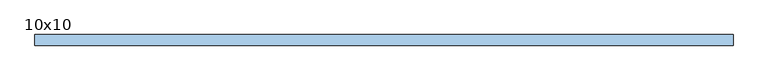
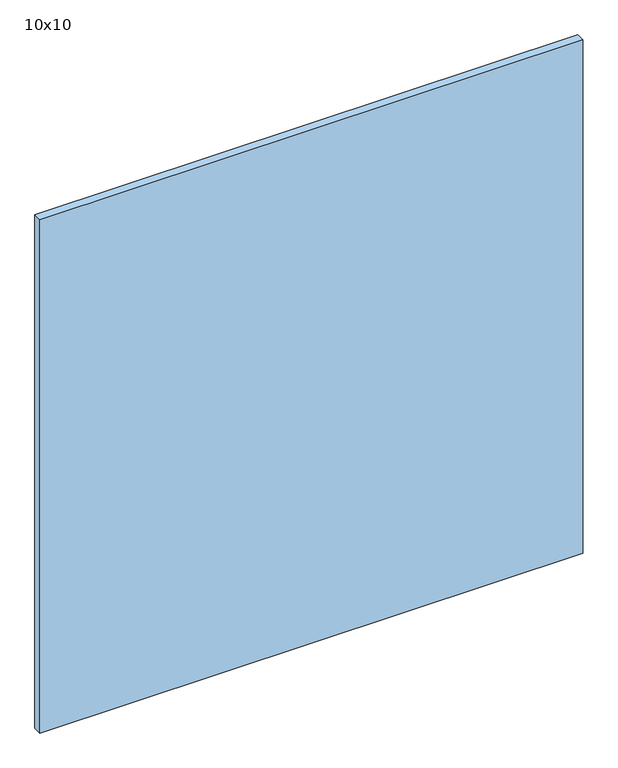
"""IFC4 building model written with IfcOpenShell, lengths in millimetres: window geometry, Window_skiss : 10x10."""

from ifc_helpers import new_model, si_unit, frame, origin, place, context, project, spatial, polyline, outline, extrude, source, transform, mapped, element, save


def window_10x10_03730955(model_context):
    return source(origin(), model_context, "Body", "SweptSolid", [
        extrude(outline(polyline([(575.0, 2.0), (-435.0, 2.0), (-435.0, 18.0), (575.0, 18.0), (575.0, 2.0)])), frame((0.0, 0.0, 800.0), z_axis=(0.0, 0.0, 1.0), x_axis=(1.0, 0.0, 0.0)), (0.0, 0.0, 1.0), 1010.0),
    ])


if __name__ == "__main__":
    model = new_model("IFC4")
    model_context = context("Model", 3, world=origin())
    ifc_project = project(units=[si_unit("LENGTHUNIT", "METRE", prefix="MILLI")], contexts=[model_context])
    site = spatial("IfcSite", under=ifc_project)
    building = spatial("IfcBuilding", under=site)
    placement = place(None, origin())
    window_10x10_shape = window_10x10_03730955(model_context)
    element("IfcWindow", 1, ObjectType="Window_skiss : 10x10", at=placement, inside=building, context=model_context, shape_type="MappedRepresentation", body=[
        mapped(window_10x10_shape, transform((0.0, 0.0, 0.0), x_axis=(1.0, 0.0, 0.0), y_axis=(0.0, 1.0, 0.0), z_axis=(0.0, 0.0, 1.0))),
    ])
    save(model, "model.ifc")

# Revit data of these elements
# Type "Window_skiss : 10x10"
#   Type Mark = "F15"
#   Keynote = "42.D"
#   Construction Type = "Generellt fönster"
#   Analytic Construction = "<None>"
#   Wall Width [instance default] = 350 mm
#   Rough Width = 1010 mm
#   Rough Height = 1010 mm
#   Inset [instance default] = 70 mm
#   Height [instance default] = 1010 mm
#   Width [instance default] = 1010 mm
#   Default Sill Height = 800 mm
#   Material Glass = Plexiglas
#   URL = ""
#   Wall Closure = (empty or 0)
#   Assembly Code = ""
# Element 1 (IfcWindow, "Window_skiss : 10x10")
#   Wall Width = 300 mm
#   Materials on its faces: "Plexiglas"
# Materials
#   "Plexiglas": class "Generic", colour RGB 201 224 223, transparency 0.85, Cost = 0
